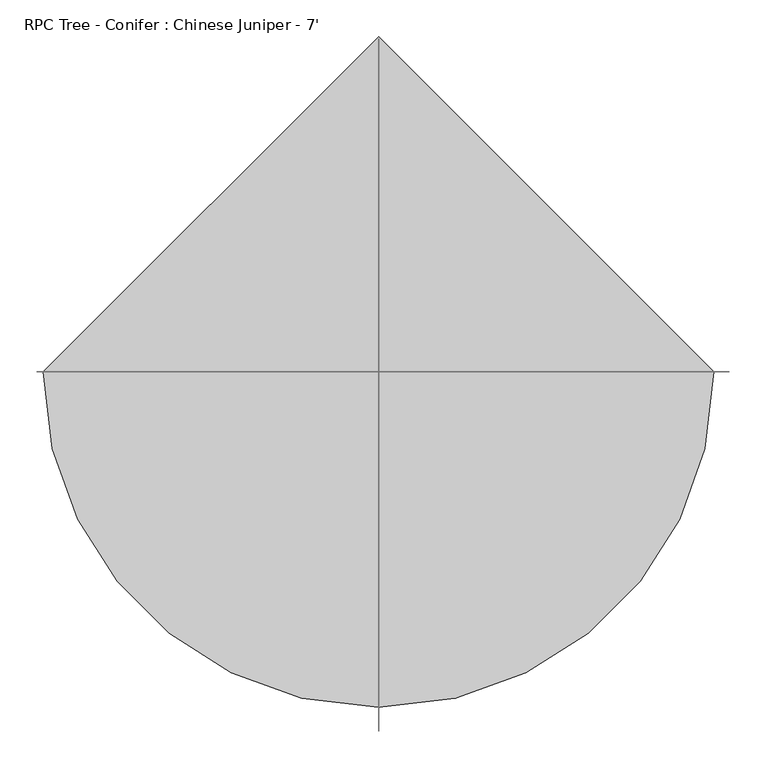
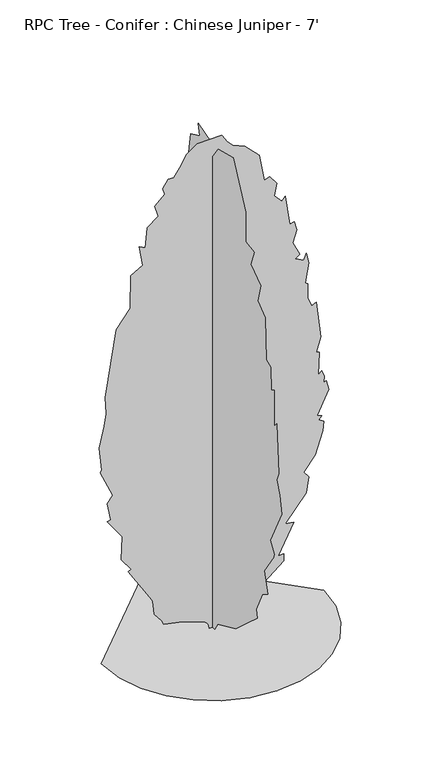
"""IFC4 building model written with IfcOpenShell, lengths in millimetres: geographic element geometry, RPC Tree - Conifer : Chinese Juniper - 7'."""

import ifcopenshell
import ifcopenshell.guid

model = None  # the IFC model being written
_history = None  # IfcOwnerHistory: only IFC2X3 demands one
_inside = {}  # id of a spatial element -> (the spatial element, [elements in it])
_under = {}  # id of a project, library or spatial element -> (it, [spatial elements below it])
_declared = {}  # id of a project -> (the project, [libraries it declares])
_typed = {}  # id of a type object -> (the type object, [elements of that type])
_made_of = {}  # id of a material, layer set ... -> (it, [elements and type objects made of it])


def new_model(schema):
    """Start an empty IFC model of exactly this schema.

    Asked for "IFC4X3", IfcOpenShell would pick the latest addendum, in which some entities
    have other attributes; the version numbers below select the first issue.
    IFC2X3 requires an IfcOwnerHistory on every rooted entity: one is made here for all.
    """
    global model, _history
    if schema == "IFC4X3":
        model = ifcopenshell.file(schema_version=(4, 3, 0, 0))
    else:
        model = ifcopenshell.file(schema=schema)
    _inside.clear()
    _under.clear()
    _declared.clear()
    _typed.clear()
    _made_of.clear()
    _history = None
    if model.schema == "IFC2X3":
        org = make("IfcOrganization", Name="unknown")
        user = make(
            "IfcPersonAndOrganization",
            ThePerson=make("IfcPerson", FamilyName="unknown"),
            TheOrganization=org,
        )
        app = make(
            "IfcApplication",
            ApplicationDeveloper=org,
            Version="unknown",
            ApplicationFullName="unknown",
            ApplicationIdentifier="unknown",
        )
        _history = make(
            "IfcOwnerHistory",
            OwningUser=user,
            OwningApplication=app,
            ChangeAction="ADDED",
            CreationDate=0,
        )
    return model


def make(cls, **values):
    """One entity of the class cls with the attributes given. An attribute that is None is left unset."""
    return model.create_entity(
        cls, **{name: value for name, value in values.items() if value is not None}
    )


def rooted(cls, **values):
    """An entity with a GlobalId (a new one), such as an element, a storey or a relation."""
    return make(cls, GlobalId=ifcopenshell.guid.new(), OwnerHistory=_history, **values)


def si_unit(unit_type, name, prefix=None):
    """IfcSIUnit, for example si_unit("LENGTHUNIT", "METRE", prefix="MILLI")."""
    return make("IfcSIUnit", UnitType=unit_type, Prefix=prefix, Name=name)


def assignment(units):
    """IfcUnitAssignment: the units of a project."""
    return None if units is None else make("IfcUnitAssignment", Units=units)


def point(xyz):
    """IfcCartesianPoint."""
    return None if xyz is None else make("IfcCartesianPoint", Coordinates=xyz)


def direction(xyz):
    """IfcDirection."""
    return None if xyz is None else make("IfcDirection", DirectionRatios=xyz)


def frame(location, z_axis=None, x_axis=None):
    """IfcAxis2Placement3D, a coordinate frame: its origin and axes. An axis left out is left unset."""
    return make(
        "IfcAxis2Placement3D",
        Location=point(location),
        Axis=direction(z_axis),
        RefDirection=direction(x_axis),
    )


def origin():
    """The frame at (0, 0, 0) with its axes left unset."""
    return frame((0.0, 0.0, 0.0))


def place(relative_to, where):
    """IfcLocalPlacement: puts the frame where relative to a parent placement (None: the world)."""
    return make(
        "IfcLocalPlacement", PlacementRelTo=relative_to, RelativePlacement=where
    )


def context(
    kind, dimensions, precision=None, world=None, true_north=None, identifier=None
):
    """IfcGeometricRepresentationContext, for example the 3D "Model" context."""
    return make(
        "IfcGeometricRepresentationContext",
        ContextIdentifier=identifier,
        ContextType=kind,
        CoordinateSpaceDimension=dimensions,
        Precision=precision,
        WorldCoordinateSystem=world,
        TrueNorth=true_north,
    )


def project(units=None, contexts=None):
    """IfcProject with its units and contexts."""
    return rooted(
        "IfcProject",
        Name="project",
        RepresentationContexts=contexts,
        UnitsInContext=assignment(units),
    )


def spatial(cls, under=None, at=None, **own):
    """A site, building, storey or space (cls), placed at a placement, below another one or the project."""
    s = rooted(cls, ObjectPlacement=at, **own)
    if under is not None:
        _under.setdefault(under.id(), (under, []))[1].append(s)
    return s


def point_list(points):
    """IfcCartesianPointList2D or 3D."""
    cls = (
        "IfcCartesianPointList2D" if len(points[0]) == 2 else "IfcCartesianPointList3D"
    )
    return make(cls, CoordList=points)


def triangles(points, corners, closed=None, point_numbers=None):
    """IfcTriangulatedFaceSet: each triangle names its three corners, points numbered from 1."""
    return make(
        "IfcTriangulatedFaceSet",
        Coordinates=point_list(points),
        Closed=closed,
        CoordIndex=corners,
        PnIndex=point_numbers,
    )


def shape(context_of_items, identifier, shape_type, items):
    """IfcShapeRepresentation: the items that make up one representation, for example the "Body"."""
    return make(
        "IfcShapeRepresentation",
        ContextOfItems=context_of_items,
        RepresentationIdentifier=identifier,
        RepresentationType=shape_type,
        Items=items,
    )


def source(mapping_origin, context_of_items, identifier, shape_type, items):
    """IfcRepresentationMap: a shape defined once, which mapped items show again and again."""
    return make(
        "IfcRepresentationMap",
        MappingOrigin=mapping_origin,
        MappedRepresentation=shape(context_of_items, identifier, shape_type, items),
    )


def transform(
    local_origin,
    x_axis=None,
    y_axis=None,
    z_axis=None,
    scale=None,
    scale2=None,
    scale3=None,
    uniform=True,
):
    """IfcCartesianTransformationOperator3D, or its non-uniform kind. x_axis, y_axis, z_axis: its Axis1, 2, 3."""
    if uniform:
        return make(
            "IfcCartesianTransformationOperator3D",
            Axis1=direction(x_axis),
            Axis2=direction(y_axis),
            LocalOrigin=point(local_origin),
            Scale=scale,
            Axis3=direction(z_axis),
        )
    return make(
        "IfcCartesianTransformationOperator3DnonUniform",
        Axis1=direction(x_axis),
        Axis2=direction(y_axis),
        LocalOrigin=point(local_origin),
        Scale=scale,
        Axis3=direction(z_axis),
        Scale2=scale2,
        Scale3=scale3,
    )


def mapped(mapping_source, mapping_target):
    """IfcMappedItem: shows the shape of a source again, moved by a transform."""
    return make(
        "IfcMappedItem", MappingSource=mapping_source, MappingTarget=mapping_target
    )


def made_of(thing, what):
    """Note that an element or type object is made of a material, layer set ...; save() writes the relation."""
    if what is not None:
        _made_of.setdefault(what.id(), (what, []))[1].append(thing)
    return thing


def element(
    cls,
    number,
    at=None,
    inside=None,
    cuts=None,
    type_object=None,
    material=None,
    context=None,
    identifier="Body",
    shape_type=None,
    held_by="IfcProductDefinitionShape",
    body=None,
    shapes=None,
    **own,
):
    """One element of the class cls, such as IfcWall. Its Tag is "e" and its number.

    at: its placement. inside: the storey or other place that contains it. cuts: it is an
    opening in that element (IfcRelVoidsElement). A single representation is given by context,
    identifier, shape_type and body (its items); several are given by shapes. held_by: the class
    of the entity that holds the representations. save() writes the other relations.
    """
    e = rooted(cls, Tag="e%d" % number, ObjectPlacement=at, **own)
    if body is not None:
        shapes = [shape(context, identifier, shape_type, body)]
    if shapes is not None:
        e.Representation = make(held_by, Representations=shapes)
    if inside is not None:
        _inside.setdefault(inside.id(), (inside, []))[1].append(e)
    if cuts is not None:
        rooted(
            "IfcRelVoidsElement", RelatingBuildingElement=cuts, RelatedOpeningElement=e
        )
    if type_object is not None:
        _typed.setdefault(type_object.id(), (type_object, []))[1].append(e)
    return made_of(e, material)


def aggregate(whole, parts):
    """IfcRelAggregates: a whole, such as a stair, and the parts it consists of."""
    return rooted("IfcRelAggregates", RelatingObject=whole, RelatedObjects=parts)


def save(model, path):
    """Write the relations noted so far, then the file.

    IfcRelAggregates (storeys below a building ...), IfcRelContainedInSpatialStructure (elements
    in a storey), IfcRelDefinesByType, IfcRelAssociatesMaterial and IfcRelDeclares: one each for
    every whole, place, type object, material and project.
    """
    for whole, parts in _under.values():
        aggregate(whole, parts)
    for where, things in _inside.values():
        rooted(
            "IfcRelContainedInSpatialStructure",
            RelatedElements=things,
            RelatingStructure=where,
        )
    for kind, things in _typed.values():
        rooted("IfcRelDefinesByType", RelatedObjects=things, RelatingType=kind)
    for what, things in _made_of.values():
        rooted("IfcRelAssociatesMaterial", RelatedObjects=things, RelatingMaterial=what)
    for by, libraries in _declared.values():
        rooted("IfcRelDeclares", RelatingContext=by, RelatedDefinitions=libraries)
    model.write(path)


def rpc_tree_conifer_chinese_juniper_7_1b9786cd(model_context):
    return source(origin(), model_context, "Body", "Tessellation", [
        triangles([(-14.517647, 6e-07, 1.3e-06), (-18.0071097, -3e-07, 17.9396969), (-27.4223632, -6e-07, 30.3914521), (-123.5685295, 1.5e-06, 65.7757953), (-201.676062, 3.9e-06, 82.3498608), (-209.1624873, 3.1e-06, 101.0656516), (-239.326362, 2.1e-06, 139.6788561), (-246.5945957, -1e-06, 198.3880905), (-257.8249785, -1.9e-06, 220.8470939), (-347.6599566, -6.4e-06, 363.0865585), (-336.0369015, -7.4e-06, 370.071561), (-375.7854927, -8.9e-06, 425.7942498), (-371.7570322, -1.5e-05, 524.6285151), (-433.7535387, -1.74e-05, 610.1379032), (-418.7802157, -1.83e-05, 613.8793173), (-433.1718882, -2.22e-05, 689.5207758), (-411.2922644, -2.49e-05, 718.6876728), (-463.6977139, -2.95e-05, 834.7279736), (-456.2123059, -3.02e-05, 842.2133451), (-467.4416714, -3.58e-05, 943.2777431), (-447.126705, -4.19e-05, 1031.4541197), (-437.4949891, -4.53e-05, 1081.7767748), (-441.2389466, -4.94e-05, 1152.8969976), (-396.3214485, -6.81e-05, 1433.6338589), (-340.174585, -7.5e-05, 1508.4981846), (-337.1392688, -8.35e-05, 1648.2265743), (-287.7691355, -8.74e-05, 1676.941246), (-302.7424948, -9.18e-05, 1763.0323574), (-277.1874594, -9.21e-05, 1748.371479), (-269.0543621, -9.76e-05, 1834.1525803), (-224.1350836, -0.0001015, 1867.8406403), (-239.107916, -0.0001038, 1916.5022049), (-197.9328675, -0.0001078, 1953.9342224), (-205.4192747, -0.000109, 1980.1369835), (-182.9602713, -0.000112, 2013.8251888), (-160.5012679, -0.000113, 2013.8251888), (-134.7328734, -0.0001161, 2047.2821583), (-108.898967, -0.0001202, 2095.8470718), (-62.5486394, -0.0001241, 2127.2339642), (37.1144179, -0.0001285, 2128.801165), (60.3458442, -0.0001273, 2092.4307106), (82.8048476, -0.000127, 2069.9720524), (132.737601, -0.0001279, 2048.8239246), (191.3566519, -0.0001268, 1987.6224277), (213.8156735, -0.0001209, 1871.5845978), (236.2746769, -0.0001223, 1879.070042), (263.6666277, -0.0001212, 1839.8828991), (254.989959, -0.0001178, 1789.2351185), (284.9366594, -0.0001171, 1755.5469131), (299.9074571, -0.0001186, 1770.5202724), (318.6248102, -0.0001119, 1643.2505699), (337.3395836, -0.0001129, 1646.9946728), (347.517378, -0.0001111, 1609.9130699), (330.7888933, -0.0001074, 1559.0291119), (359.7983145, -0.000105, 1497.2687828), (340.1843954, -0.0001034, 1485.5084541), (374.7716738, -0.0001038, 1467.3220642), (386.0010392, -0.0001059, 1493.5248253), (397.230441, -0.0001037, 1448.6072182), (382.2596251, -9.81e-05, 1366.2577389), (393.0673594, -9.81e-05, 1357.3651131), (391.5662155, -9.44e-05, 1296.562429), (408.4598064, -9.28e-05, 1257.7053532), (427.1771233, -9.41e-05, 1265.1907974), (445.8918966, -8.55e-05, 1107.9794632), (427.1771233, -8.11e-05, 1048.0886421), (438.8332068, -8.14e-05, 1044.1287821), (434.6625312, -7.54e-05, 947.0217007), (449.6358905, -7.68e-05, 958.2511024), (460.8652559, -7.57e-05, 932.0483414), (457.1212984, -7.4e-05, 905.8481964), (468.3506639, -7.47e-05, 909.5896105), (479.5800293, -7.27e-05, 868.4161062), (430.9185737, -6.48e-05, 771.0931223), (449.6358905, -6.52e-05, 763.6077507), (438.4064887, -6.38e-05, 748.6343914), (457.1212984, -6.39e-05, 737.4049896), (453.1842567, -6.13e-05, 697.0620306), (423.4331657, -5.44e-05, 602.6499518), (374.7716738, -4.87e-05, 542.7590944), (397.230441, -4.81e-05, 516.5563697), (384.9545551, -4.37e-05, 451.166393), (299.9074571, -3.36e-05, 344.3717488), (333.5981332, -3.49e-05, 340.6277913), (269.9633001, -2.47e-05, 217.1038994), (292.4220673, -2.57e-05, 217.1038994), (292.4220673, -2.39e-05, 187.1584707), (127.7223548, -8.7e-06, 52.4044321), (127.7223548, -9.8e-06, 71.1202274), (15.4277284, -7e-07, 0.0), (0.1966721, 13.7891713, 0.00013), (0.1966737, 34.4811189, 14.2963339), (0.1966762, 77.4229995, 29.9456808), (0.1966783, 178.488651, 67.3772736), (0.1966827, 230.8930831, 116.0384931), (0.1966819, 208.4340797, 119.7817057), (0.1966904, 288.5449239, 235.2565704), (0.1966918, 264.5824875, 291.9663175), (0.196695, 331.9587347, 389.2892833), (0.1966967, 324.4733268, 434.2067814), (0.1967014, 373.1322753, 494.0976388), (0.1967052, 389.4924685, 565.7309481), (0.1967041, 380.6202267, 640.0820784), (0.1967106, 440.5110841, 729.9170746), (0.1967147, 444.2524981, 819.7546143), (0.196717, 422.6319428, 893.2725832), (0.1967196, 455.4818636, 1010.6565519), (0.19672, 425.5377248, 1051.8300562), (0.1967236, 388.1056346, 1171.611771), (0.1967244, 414.3083593, 1253.9613956), (0.1967283, 384.3616407, 1373.7430378), (0.1967298, 346.932094, 1444.8632607), (0.1967315, 328.2147772, 1594.5917667), (0.19673, 305.75601, 1583.362365), (0.1967359, 305.75601, 1718.1148956), (0.1967344, 260.8385118, 1729.3441521), (0.1967329, 237.0752094, 1809.303661), (0.1967352, 223.406676, 1875.3287006), (0.1967352, 178.488651, 1920.2461624), (0.1967401, 156.0296476, 2055.0011639), (0.1967346, 92.3955867, 2084.9454117), (0.1967371, 102.0598133, 2133.1292439), (0.1967319, 11.3487565, 2104.2112415), (0.1967329, 6.3027505, 2040.0278046), (0.1967297, -38.6152347, 2103.6627285), (0.1967262, -147.1670527, 2133.606831), (0.1967183, -237.0033388, 1950.1902649), (0.1967127, -237.0033388, 1822.9231785), (0.1967097, -296.2055936, 1812.3847229), (0.1967078, -270.691199, 1744.3175114), (0.1967065, -342.8426634, 1695.0642677), (0.196704, -323.0966666, 1617.050425), (0.1966999, -375.4995727, 1575.8744499), (0.1966957, -382.9874877, 1396.2018414), (0.1966938, -413.5488853, 1383.1639744), (0.1966894, -416.6756204, 1283.9081142), (0.196689, -439.1343876, 1298.8788574), (0.1966862, -439.1343876, 1141.6675959), (0.1966823, -457.849161, 1164.1263994), (0.1966765, -472.8225203, 954.5096884), (0.1966757, -456.5690065, 918.855542), (0.1966723, -480.3104716, 864.672076), (0.1966725, -491.5398371, 789.8078957), (0.1966689, -412.9316628, 628.8526766), (0.1966658, -439.1343876, 583.9351785), (0.1966692, -436.9195155, 568.0778978), (0.1966679, -368.0141647, 467.8974212), (0.1966629, -394.2168895, 381.8038754), (0.1966636, -353.0408054, 355.6011506), (0.1966655, -311.8672648, 265.7661362), (0.1966637, -319.3526728, 232.0767318), (0.196664, -244.4894916, 164.6997216), (0.1966643, -165.8828434, 93.5794897), (0.1966675, -34.8715179, 33.6886368), (0.1966708, -16.1562041, 0.0001282), (-457.9674314, 0.0, 0.0001492), (-445.8541446, -104.9808196, 0.0001424), (-411.358285, -201.3891246, 0.0001352), (-357.2408761, -286.4621113, 0.0001277), (-286.2654482, -357.4375574, 0.0001204), (-201.1924614, -411.5549664, 0.0001134), (-104.7841473, -446.0508259, 0.0001072), (0.1966917, -458.1641127, 0.0001019), (105.1774918, -446.0508259, 9.8e-05), (201.5857877, -411.5549664, 9.58e-05), (286.6587745, -357.4375574, 9.54e-05), (357.6342387, -286.4621113, 9.65e-05), (411.7516477, -201.3888702, 9.92e-05), (446.2475072, -104.9808196, 0.0001034), (458.360794, 4.01e-05, 0.0001092), (0.1966112, 458.1641127, 0.0001565)], [[57, 58, 59], [27, 28, 29], [87, 88, 89], [49, 50, 51], [13, 14, 15], [83, 84, 85], [74, 75, 76], [63, 64, 65], [68, 69, 70], [71, 72, 73], [9, 10, 11], [85, 86, 87], [85, 87, 89], [51, 52, 53], [54, 55, 56], [90, 1, 2], [66, 67, 68], [45, 46, 47], [17, 18, 19], [68, 70, 71], [45, 47, 48], [31, 32, 33], [76, 77, 78], [89, 90, 2], [89, 2, 3], [57, 59, 60], [51, 53, 54], [25, 26, 27], [39, 40, 41], [56, 57, 60], [71, 73, 74], [34, 35, 36], [33, 34, 36], [4, 5, 6], [60, 61, 62], [80, 81, 82], [38, 39, 41], [37, 38, 41], [37, 41, 42], [29, 30, 31], [15, 16, 17], [36, 37, 42], [33, 36, 42], [31, 33, 42], [31, 42, 43], [31, 43, 44], [31, 44, 45], [29, 31, 45], [29, 45, 48], [27, 29, 48], [25, 27, 48], [25, 48, 49], [25, 49, 51], [25, 51, 54], [25, 54, 56], [25, 56, 60], [25, 60, 62], [24, 25, 62], [23, 24, 62], [22, 23, 62], [22, 62, 63], [22, 63, 65], [22, 65, 66], [22, 66, 68], [21, 22, 68], [20, 21, 68], [19, 20, 68], [17, 19, 68], [17, 68, 71], [17, 71, 74], [15, 17, 74], [13, 15, 74], [13, 74, 76], [13, 76, 78], [13, 78, 79], [13, 79, 80], [12, 13, 80], [11, 12, 80], [9, 11, 80], [9, 80, 82], [9, 82, 83], [9, 83, 85], [9, 85, 89], [9, 89, 3], [9, 3, 4], [8, 9, 4], [8, 4, 6], [7, 8, 6], [138, 139, 140], [94, 95, 96], [136, 137, 138], [121, 122, 123], [112, 113, 114], [128, 129, 130], [121, 123, 124], [125, 126, 127], [124, 125, 127], [114, 115, 116], [147, 148, 149], [130, 131, 132], [124, 127, 128], [134, 135, 136], [154, 155, 91], [154, 91, 92], [150, 151, 152], [96, 97, 98], [119, 120, 121], [119, 121, 124], [119, 124, 128], [118, 119, 128], [117, 118, 128], [116, 117, 128], [116, 128, 130], [114, 116, 130], [114, 130, 132], [112, 114, 132], [112, 132, 133], [112, 133, 134], [112, 134, 136], [111, 112, 136], [110, 111, 136], [109, 110, 136], [109, 136, 138], [109, 138, 140], [109, 140, 141], [108, 109, 141], [107, 108, 141], [106, 107, 141], [105, 106, 141], [104, 105, 141], [103, 104, 141], [103, 141, 142], [103, 142, 143], [103, 143, 144], [102, 103, 144], [101, 102, 144], [100, 101, 144], [100, 144, 145], [100, 145, 146], [100, 146, 147], [100, 147, 149], [100, 149, 150], [100, 150, 152], [100, 152, 153], [100, 153, 154], [99, 100, 154], [98, 99, 154], [96, 98, 154], [96, 154, 92], [96, 92, 93], [96, 93, 94], [170, 171, 156], [169, 170, 156], [169, 156, 157], [168, 169, 157], [168, 157, 158], [168, 158, 159], [167, 168, 159], [166, 167, 159], [166, 159, 160], [166, 160, 161], [166, 161, 162], [166, 162, 163], [166, 163, 164], [166, 164, 165]], closed=False),
    ])


if __name__ == "__main__":
    model = new_model("IFC4")
    model_context = context("Model", 3, world=origin())
    ifc_project = project(units=[si_unit("LENGTHUNIT", "METRE", prefix="MILLI")], contexts=[model_context])
    site = spatial("IfcSite", under=ifc_project)
    building = spatial("IfcBuilding", under=site)
    placement = place(None, origin())
    rpc_tree_conifer_chinese_juniper_7_shape = rpc_tree_conifer_chinese_juniper_7_1b9786cd(model_context)
    element("IfcGeographicElement", 1, ObjectType="RPC Tree - Conifer : Chinese Juniper - 7'", at=placement, inside=building, context=model_context, shape_type="MappedRepresentation", body=[
        mapped(rpc_tree_conifer_chinese_juniper_7_shape, transform((0.0, 0.0, 0.0), x_axis=(1.0, 0.0, 0.0), y_axis=(0.0, 1.0, 0.0), z_axis=(0.0, 0.0, 1.0))),
    ])
    save(model, "model.ifc")

# Revit data of these elements
# Type "RPC Tree - Conifer : Chinese Juniper - 7'"
#   built-in parameter 1005198 = "{2, 15},{39, RPC-16-FUM3-UUQ0-UBF0-N000-ST1L-LVER-AU},{1, 0},{1, 0},{2, 35},{1, 8},{5, Color},{1, 0},{1, 0},{3, 0.8},{3, 0.8},{3, 0.8},{1, 8},{7, BBoxMin},{1, 0},{1, 0},{1, 0},{1, 0},{1, 0},{1, 8},{7, BBoxMax},{1, 0},{1, 0},{1, 0},{1, 0},{1, 0},{2, 11},{9, RPCTypeId},{1, 0},{1, 0},{39, RPC-16-FUM3-UUQ0-UBF0-N000-ST1L-LVER-AU},{1, 6},{14, RPCPlantHeight},{1, 0},{1, 0},{1, 7},{2, 11},{7, keyword},{1, 0},{1, 0},{96, :Geometry:RPC:Chinese Juniper:juniperus chinensis:chinese:juniper:cupressaceae:conifer:evergreen},{2, 11},{8, category},{1, 0},{1, 0},{16, :Trees [General]},{2, 11},{12, LocalizedUID},{1, 0},{1, 0},{15, Chinese Juniper},{2, 14},{6, Height},{1, 0},{1, 0},{1, 7},{1, 2},{16, Cast Reflections},{1, 0},{1, 0},{1, 0},{1, 2},{12, Cast Shadows},{1, 0},{1, 0},{1, 1},{1, 2},{9, Lock View},{1, 0},{1, 0},{1, 0},{1, 4},{5, ViewC},{1, 0},{1, 0},{1, 0},{2, 11},{20, AdvancedUIDefinition},{1, 0},{1, 0},{0, },{2, 11},{10, AssetLibID},{1, 0},{1, 0},{36, 4D3F6E72-3F99-4203-98E9-AF80B3C7A7A4},{2, 11},{10, BaseSchema},{1, 0},{1, 0},{9, RPCSchema},{2, 11},{12, ExchangeGUID},{1, 0},{1, 0},{0, },{1, 2},{6, Hidden},{1, 0},{1, 0},{1, 0},{1, 4},{11, RPCCategory},{1, 0},{1, 0},{1, 0},{2, 11},{8, RPCImage},{1, 0},{1, 0},{0, },{1, 4},{13, SchemaVersion},{1, 0},{1, 0},{1, 4},{2, 11},{12, UIDefinition},{1, 0},{1, 0},{0, },{2, 11},{6, UIName},{1, 0},{1, 0},{39, RPC-16-FUM3-UUQ0-UBF0-N000-ST1L-LVER-AU},{2, 11},{11, VersionGUID},{1, 0},{1, 0},{9, RPCSchema},{2, 11},{9, assettype},{1, 0},{1, 0},{11, RPCGeometry},{2, 11},{11, description},{1, 0},{1, 0},{0, },{2, 11},{9, localname},{1, 0},{1, 0},{3, RPC},{2, 11},{9, localtype},{1, 0},{1, 0},{3, RPC},{1, 4},{8, revision},{1, 0},{1, 0},{1, 1},{2, 11},{9, thumbnail},{1, 0},{1, 0},{0, },{1, 4},{7, version},{1, 0},{1, 0},{1, 1},{1, 2},{20, RPC_Cast Reflections},{1, 0},{1, 0},{1, 1},{1, 2},{16, RPC_Cast Shadows},{1, 0},{1, 0},{1, 1},{1, 2},{13, RPC_Lock View},{1, 0},{1, 0},{1, 0},{1, 4},{9, RPC_ViewC},{1, 0},{1, 0},{1, 0},{21, assetlibrary_base.fbx},{1, 5},"
#   built-in parameter 1005195 = "RPC-16-FUM3-UUQ0-UBF0-N000-ST1L-LVER-AU"
#   Type Comments = "Chinese Juniper"
#   Assembly Code = "G2050500"
#   Height = 213.36 cm
#   Description = (empty or 0)
#   Default Elevation = 0
